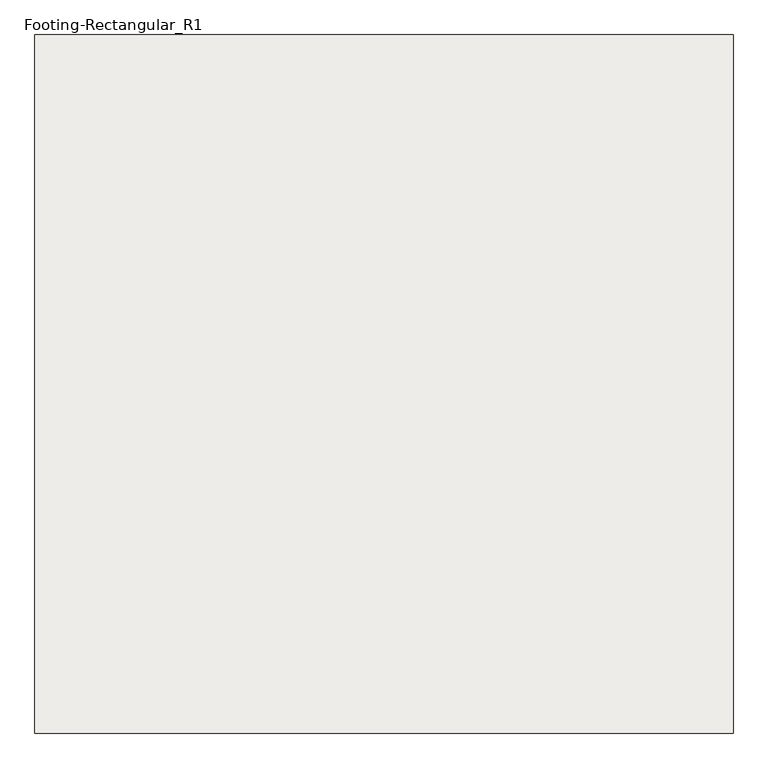
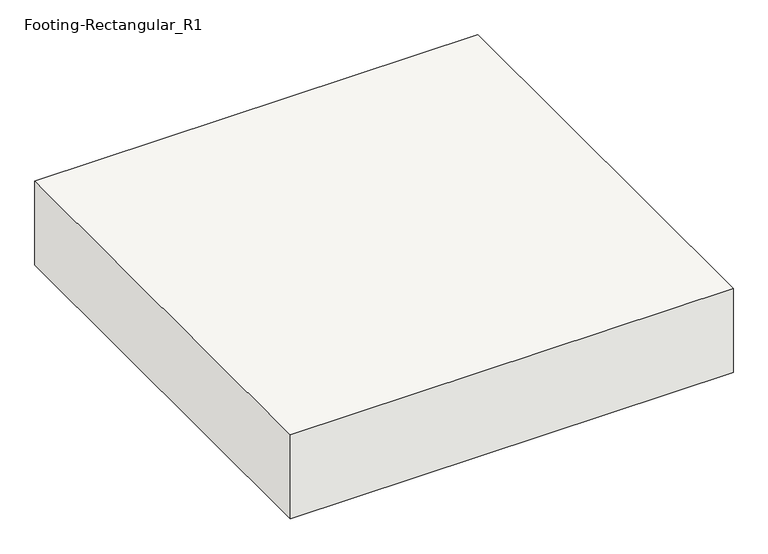
"""IFC4 building model written with IfcOpenShell, lengths in millimetres: slab geometry, Footing-Rectangular_R1 : H_SF_AR_S18_W2500xL2500xT500_Bitumen_F1."""

from ifc_helpers import new_model, si_unit, frame, origin, place, context, project, spatial, polyline, outline, extrude, source, transform, mapped, element, save


def footing_rectangular_r1_513089b3(model_context):
    return source(origin(), model_context, "Body", "SweptSolid", [
        extrude(outline(polyline([(1250.0, 1250.0), (1250.0, -1250.0), (-1250.0, -1250.0), (-1250.0, 1250.0), (1250.0, 1250.0)])), frame((0.0, 0.0, -500.0), z_axis=(0.0, 0.0, 1.0), x_axis=(1.0, 0.0, 0.0)), (0.0, 0.0, 1.0), 500.0),
    ])


if __name__ == "__main__":
    model = new_model("IFC4")
    model_context = context("Model", 3, world=origin())
    ifc_project = project(units=[si_unit("LENGTHUNIT", "METRE", prefix="MILLI")], contexts=[model_context])
    site = spatial("IfcSite", under=ifc_project)
    building = spatial("IfcBuilding", under=site)
    placement = place(None, origin())
    footing_rectangular_r1_shape = footing_rectangular_r1_513089b3(model_context)
    element("IfcSlab", 1, ObjectType="Footing-Rectangular_R1 : H_SF_AR_S18_W2500xL2500xT500_Bitumen_F1", at=placement, inside=building, context=model_context, shape_type="MappedRepresentation", body=[
        mapped(footing_rectangular_r1_shape, transform((0.0, 0.0, 0.0), x_axis=(1.0, 0.0, 0.0), y_axis=(0.0, 1.0, 0.0), z_axis=(0.0, 0.0, 1.0))),
    ])
    save(model, "model.ifc")

# Revit data of these elements
# Type "Footing-Rectangular_R1 : H_SF_AR_S18_W2500xL2500xT500_Bitumen_F1"
#   Type Mark = "F1"
#   Top bar = "D25@300"
#   Description = "UG Shallow Foundation"
#   Bottom bar = "D20@300"
#   Width = 2500 mm
#   Length = 2500 mm
#   Foundation Thickness = 500 mm
#   Structural Material [instance default] = none
#   Assembly Code = ""
